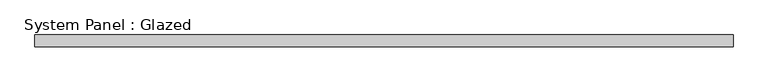
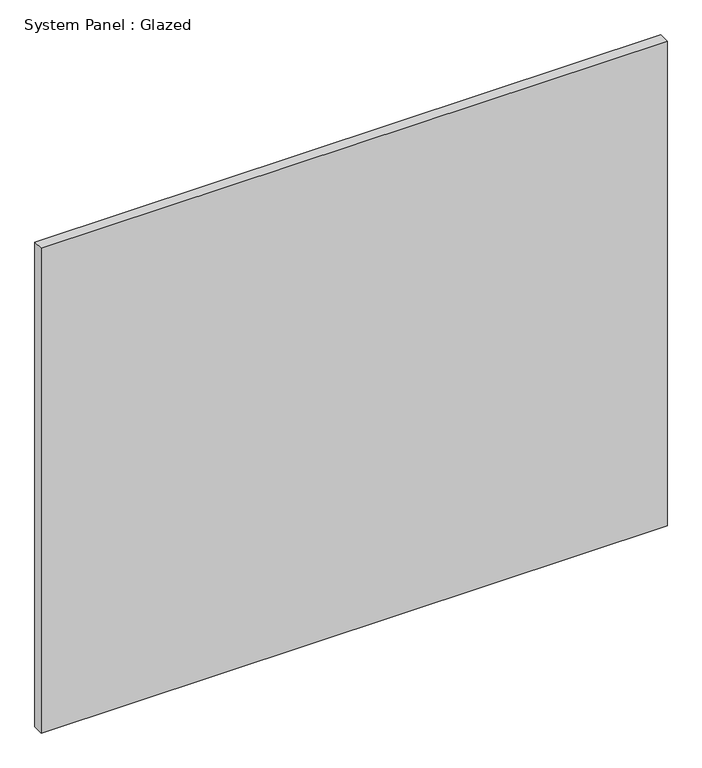
"""IFC4 building model written with IfcOpenShell, lengths in millimetres: plate geometry, System Panel : Glazed."""

from ifc_helpers import new_model, si_unit, origin, origin_with_axes, place, context, project, spatial, polyline, outline, extrude, source, transform, mapped, element, save


def system_panel_glazed_a326aec2(model_context):
    return source(origin(), model_context, "Body", "SweptSolid", [
        extrude(outline(polyline([(732.9083116, 24.5), (-732.9083116, 24.5), (-732.9083116, 49.5), (732.9083116, 49.5), (732.9083116, 24.5)])), origin_with_axes(), (0.0, 0.0, 1.0), 1200.0),
    ])


if __name__ == "__main__":
    model = new_model("IFC4")
    model_context = context("Model", 3, world=origin())
    ifc_project = project(units=[si_unit("LENGTHUNIT", "METRE", prefix="MILLI")], contexts=[model_context])
    site = spatial("IfcSite", under=ifc_project)
    building = spatial("IfcBuilding", under=site)
    placement = place(None, origin())
    system_panel_glazed_shape = system_panel_glazed_a326aec2(model_context)
    element("IfcPlate", 1, ObjectType="System Panel : Glazed", at=placement, inside=building, context=model_context, shape_type="MappedRepresentation", body=[
        mapped(system_panel_glazed_shape, transform((0.0, 0.0, 0.0), x_axis=(1.0, 0.0, 0.0), y_axis=(0.0, 1.0, 0.0), z_axis=(0.0, 0.0, 1.0))),
    ])
    save(model, "model.ifc")

# Revit data of these elements
# Element 1 (IfcPlate, "System Panel : Glazed")
#   Materials on its faces: "Glass"
# Materials
#   "Glass": class "Glass", colour RGB 218 227 224, transparency 0.85, Description = "Soda Lime Glass", Cost = 0
